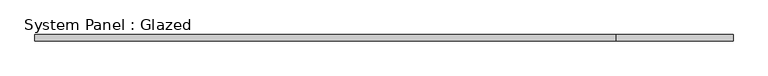
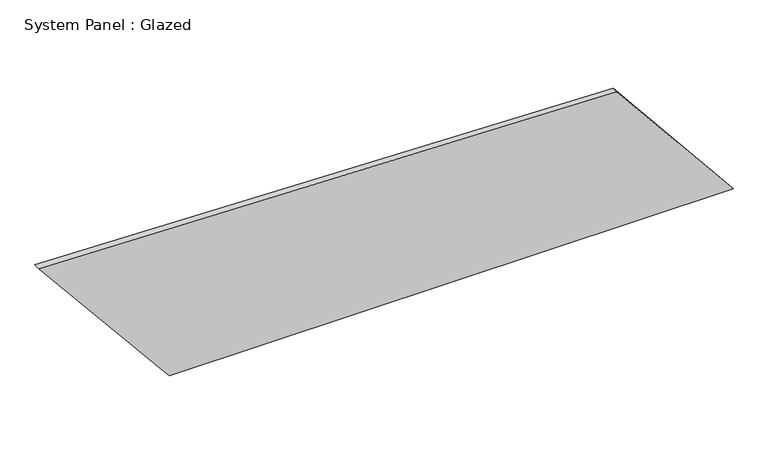
"""IFC4 building model written with IfcOpenShell, lengths in millimetres: plate geometry, System Panel : Glazed."""

from ifc_helpers import new_model, si_unit, frame, origin, place, context, project, spatial, polyline, outline, extrude, source, transform, mapped, element, save


def system_panel_glazed_7f5d6e41(model_context):
    return source(origin(), model_context, "Body", "SweptSolid", [
        extrude(outline(polyline([(0.0, -867.9725866), (0.0, 1390.391356), (573.7376077, 925.180396), (636.5848398, -1390.391356), (0.0, -867.9725866)])), frame((0.0, -49.5, 0.0), z_axis=(0.0, 1.0, 0.0), x_axis=(0.0, 0.0, 1.0)), (0.0, 0.0, 1.0), 25.0),
    ])


if __name__ == "__main__":
    model = new_model("IFC4")
    model_context = context("Model", 3, world=origin())
    ifc_project = project(units=[si_unit("LENGTHUNIT", "METRE", prefix="MILLI")], contexts=[model_context])
    site = spatial("IfcSite", under=ifc_project)
    building = spatial("IfcBuilding", under=site)
    placement = place(None, origin())
    system_panel_glazed_shape = system_panel_glazed_7f5d6e41(model_context)
    element("IfcPlate", 1, ObjectType="System Panel : Glazed", at=placement, inside=building, context=model_context, shape_type="MappedRepresentation", body=[
        mapped(system_panel_glazed_shape, transform((0.0, 0.0, 0.0), x_axis=(1.0, 0.0, 0.0), y_axis=(0.0, 1.0, 0.0), z_axis=(0.0, 0.0, 1.0))),
    ])
    save(model, "model.ifc")

# Revit data of these elements
# Element 1 (IfcPlate, "System Panel : Glazed")
#   Materials on its faces: "Glass, Clear Glazing"
# Materials
#   "Glass, Clear Glazing": class "Glass", colour RGB 247 249 248, transparency 0.85, Description = "Clear glazing", Cost = 0
